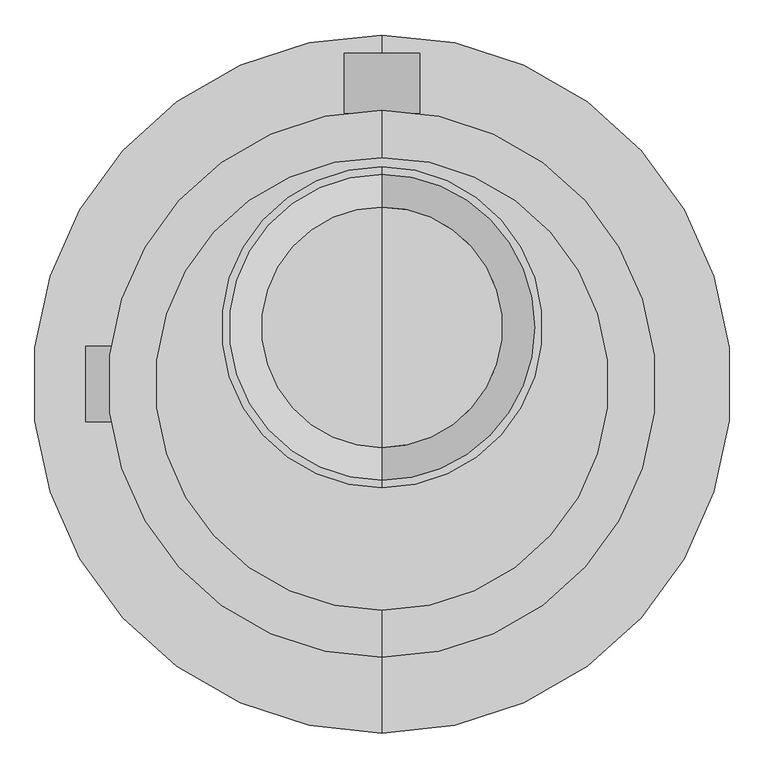
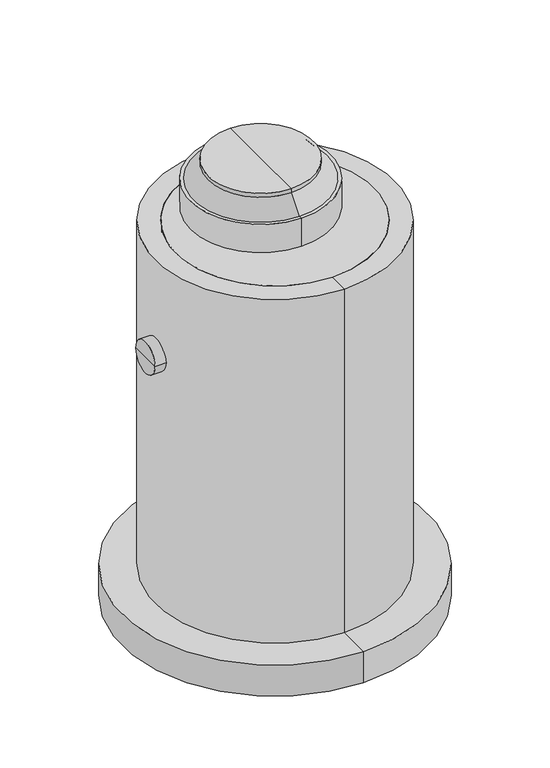
"""IFC4 building model written with IfcOpenShell, lengths in millimetres: proxy geometry, Stormceptor STC - 450 : Stormceptor STC - 450."""

from ifc_helpers import new_model, si_unit, point, frame, origin, origin_2d, place, context, project, spatial, polyline, circle_curve, trimmed, segment, composite_curve, outline, extrude, source, transform, mapped, element, save
from ifc_brep_helpers import plane_surface, cylinder_surface, revolved_surface, advanced_brep


def generic_models_1f94928f(model_context):
    return source(origin(), model_context, "Body", "SolidModel", [
        advanced_brep(
        [(-600.2627198, -101.6, 1828.8), (-600.2627198, 101.6, 1828.8), (-600.2627198, 0.0, 1828.8), (-797.6860951, -101.6, 1828.8), (-797.6860951, 101.6, 1828.8), (-797.6860951, 0.0, 1828.8)],
        [
            (0, 1, circle_curve(frame((-600.2627198, 0.0, 1828.8), z_axis=(1.0, 0.0, 0.0), x_axis=(0.0, 1.0, 0.0)), 101.6)),
            (1, 2),
            (2, 0),
            (1, 0, circle_curve(frame((-600.2627198, 0.0, 1828.8), z_axis=(1.0, 0.0, 0.0), x_axis=(0.0, 1.0, 0.0)), 101.6)),
            (3, 4, circle_curve(frame((-797.6860951, 0.0, 1828.8), z_axis=(1.0, 0.0, 0.0), x_axis=(0.0, 1.0, 0.0)), 101.6)),
            (4, 1),
            (0, 3),
            (4, 3, circle_curve(frame((-797.6860951, 0.0, 1828.8), z_axis=(1.0, 0.0, 0.0), x_axis=(0.0, 1.0, 0.0)), 101.6)),
            (5, 4),
            (3, 5),
        ],
        [
            plane_surface(frame((-600.2627198, 0.0, 1828.8), z_axis=(1.0, 0.0, 0.0), x_axis=(0.0, 1.0, 0.0))),
            cylinder_surface(frame((-1135.9594561, 0.0, 1828.8), z_axis=(-1.0, 0.0, 0.0), x_axis=(0.0, 1.0, 0.0)), 101.6),
            plane_surface(frame((-797.6860951, 0.0, 1828.8), z_axis=(-1.0, 0.0, 0.0), x_axis=(0.0, 1.0, 0.0))),
        ],
        [
            (0, [[1, 2, 3]]),
            (0, [[4, -3, -2]]),
            (1, [[5, 6, -1, 7]]),
            (1, [[8, -7, -4, -6]]),
            (2, [[9, -5, 10]]),
            (2, [[-10, -8, -9]]),
        ],
    ),
        advanced_brep(
        [(-101.6, 729.5594561, 1905.0), (101.6, 729.5594561, 1905.0), (0.0, 729.5594561, 1905.0), (-101.6, 890.1336251, 1905.0), (101.6, 890.1336251, 1905.0), (0.0, 890.1336251, 1905.0)],
        [
            (0, 1, circle_curve(frame((0.0, 729.5594561, 1905.0), z_axis=(0.0, -1.0, 0.0), x_axis=(1.0, 0.0, 0.0)), 101.6)),
            (1, 2),
            (2, 0),
            (1, 0, circle_curve(frame((0.0, 729.5594561, 1905.0), z_axis=(0.0, -1.0, 0.0), x_axis=(1.0, 0.0, 0.0)), 101.6)),
            (3, 4, circle_curve(frame((0.0, 890.1336251, 1905.0), z_axis=(0.0, -1.0, 0.0), x_axis=(1.0, 0.0, 0.0)), 101.6)),
            (4, 1),
            (0, 3),
            (4, 3, circle_curve(frame((0.0, 890.1336251, 1905.0), z_axis=(0.0, -1.0, 0.0), x_axis=(1.0, 0.0, 0.0)), 101.6)),
            (5, 4),
            (3, 5),
        ],
        [
            plane_surface(frame((0.0, 729.5594561, 1905.0), z_axis=(0.0, -1.0, 0.0), x_axis=(1.0, 0.0, 0.0))),
            cylinder_surface(frame((0.0, 805.7594561, 1905.0), z_axis=(0.0, 1.0, 0.0), x_axis=(1.0, 0.0, 0.0)), 101.6),
            plane_surface(frame((0.0, 890.1336251, 1905.0), z_axis=(0.0, 1.0, 0.0), x_axis=(1.0, 0.0, 0.0))),
        ],
        [
            (0, [[1, 2, 3]]),
            (0, [[4, -3, -2]]),
            (1, [[5, 6, -1, 7]]),
            (1, [[8, -7, -4, -6]]),
            (2, [[9, -5, 10]]),
            (2, [[-10, -8, -9]]),
        ],
    ),
        extrude(outline(composite_curve([segment(trimmed(circle_curve(origin_2d(), 609.6), [point((0.0, -609.6))], [point((0.0, 609.6))], False, "CARTESIAN"), True, "CONTINUOUS"), segment(trimmed(circle_curve(origin_2d(), 609.6), [point((0.0, 609.6))], [point((0.0, -609.6))], False, "CARTESIAN"), True, "CONTINUOUS")], self_intersect=False)), frame((0.0, 0.0, 2235.2), z_axis=(0.0, 0.0, 1.0), x_axis=(1.0, 0.0, 0.0)), (0.0, 0.0, 1.0), 203.2),
        advanced_brep(
        [(0.0, 584.2, 2621.28), (0.0, -279.4, 2621.28), (0.0, 152.4, 2621.28), (0.0, 584.2, 2438.4), (0.0, -279.4, 2438.4), (0.0, 152.4, 2438.4)],
        [
            (0, 1, circle_curve(frame((0.0, 152.4, 2621.28), z_axis=(0.0, 0.0, 1.0), x_axis=(0.0, -1.0, 0.0)), 431.8)),
            (1, 2),
            (2, 0),
            (1, 0, circle_curve(frame((0.0, 152.4, 2621.28), z_axis=(0.0, 0.0, 1.0), x_axis=(0.0, -1.0, 0.0)), 431.8)),
            (3, 4, circle_curve(frame((0.0, 152.4, 2438.4), z_axis=(0.0, 0.0, 1.0), x_axis=(0.0, -1.0, 0.0)), 431.8)),
            (4, 1),
            (0, 3),
            (4, 3, circle_curve(frame((0.0, 152.4, 2438.4), z_axis=(0.0, 0.0, 1.0), x_axis=(0.0, -1.0, 0.0)), 431.8)),
            (5, 4),
            (3, 5),
        ],
        [
            plane_surface(frame((0.0, 152.4, 2621.28), z_axis=(0.0, 0.0, 1.0), x_axis=(0.0, -1.0, 0.0))),
            cylinder_surface(frame((0.0, 152.4, 2529.84), z_axis=(0.0, 0.0, -1.0), x_axis=(0.0, -1.0, 0.0)), 431.8),
            plane_surface(frame((0.0, 152.4, 2438.4), z_axis=(0.0, 0.0, -1.0), x_axis=(0.0, -1.0, 0.0))),
        ],
        [
            (0, [[1, 2, 3]]),
            (0, [[4, -3, -2]]),
            (1, [[5, 6, -1, 7]]),
            (1, [[8, -7, -4, -6]]),
            (2, [[9, -5, 10]]),
            (2, [[-10, -8, -9]]),
        ],
    ),
        advanced_brep(
        [(0.0, 609.6, 203.2), (0.0, -609.6, 203.2), (0.0, -736.6, 203.2), (0.0, 736.6, 203.2), (0.0, 609.6, 2438.4), (0.0, -609.6, 2438.4), (0.0, 736.6, 2438.4), (0.0, -736.6, 2438.4)],
        [
            (0, 1, circle_curve(frame((0.0, 0.0, 203.2), z_axis=(0.0, 0.0, 1.0), x_axis=(0.0, -1.0, 0.0)), 609.6)),
            (1, 2),
            (2, 3, circle_curve(frame((0.0, 0.0, 203.2), z_axis=(0.0, 0.0, -1.0), x_axis=(0.0, -1.0, 0.0)), 736.6)),
            (3, 0),
            (1, 0, circle_curve(frame((0.0, 0.0, 203.2), z_axis=(0.0, 0.0, 1.0), x_axis=(0.0, -1.0, 0.0)), 609.6)),
            (3, 2, circle_curve(frame((0.0, 0.0, 203.2), z_axis=(0.0, 0.0, -1.0), x_axis=(0.0, -1.0, 0.0)), 736.6)),
            (4, 5, circle_curve(frame((0.0, 0.0, 2438.4), z_axis=(0.0, 0.0, 1.0), x_axis=(0.0, -1.0, 0.0)), 609.6)),
            (5, 1),
            (0, 4),
            (5, 4, circle_curve(frame((0.0, 0.0, 2438.4), z_axis=(0.0, 0.0, 1.0), x_axis=(0.0, -1.0, 0.0)), 609.6)),
            (6, 7, circle_curve(frame((0.0, 0.0, 2438.4), z_axis=(0.0, 0.0, 1.0), x_axis=(0.0, -1.0, 0.0)), 736.6)),
            (7, 5),
            (4, 6),
            (7, 6, circle_curve(frame((0.0, 0.0, 2438.4), z_axis=(0.0, 0.0, 1.0), x_axis=(0.0, -1.0, 0.0)), 736.6)),
            (2, 7),
            (6, 3),
        ],
        [
            plane_surface(frame((0.0, 0.0, 203.2), z_axis=(0.0, 0.0, -1.0), x_axis=(0.0, -1.0, 0.0))),
            revolved_surface(polyline([(0.0, -609.6, 203.2), (0.0, -609.6, 2438.4)]), (0.0, 0.0, 431.8), (0.0, 0.0, -1.0)),
            plane_surface(frame((0.0, 0.0, 2438.4), z_axis=(0.0, 0.0, 1.0), x_axis=(0.0, -1.0, 0.0))),
            cylinder_surface(frame((0.0, 0.0, 431.8), z_axis=(0.0, 0.0, -1.0), x_axis=(0.0, -1.0, 0.0)), 736.6),
        ],
        [
            (0, [[1, 2, 3, 4]]),
            (0, [[5, -4, 6, -2]]),
            (1, [[7, 8, -1, 9]]),
            (1, [[10, -9, -5, -8]]),
            (2, [[11, 12, -7, 13]]),
            (2, [[14, -13, -10, -12]]),
            (3, [[-3, 15, -11, 16]]),
            (3, [[-6, -16, -14, -15]]),
        ],
    ),
        advanced_brep(
        [(0.0, -171.45, 2722.88), (0.0, 476.25, 2722.88), (0.0, 564.5695326, 2621.28), (0.0, -259.7695326, 2621.28), (0.0, -171.45, 2748.28), (0.0, 476.25, 2748.28), (0.0, 152.4, 2748.28), (0.0, 152.4, 2621.28)],
        [
            (0, 1, circle_curve(frame((0.0, 152.4, 2722.88), z_axis=(0.0, 0.0, -1.0), x_axis=(0.0, 1.0, 0.0)), 323.85)),
            (1, 2),
            (2, 3, circle_curve(frame((0.0, 152.4, 2621.28), z_axis=(0.0, 0.0, 1.0), x_axis=(0.0, 1.0, 0.0)), 412.1695326)),
            (3, 0),
            (1, 0, circle_curve(frame((0.0, 152.4, 2722.88), z_axis=(0.0, 0.0, -1.0), x_axis=(0.0, 1.0, 0.0)), 323.85)),
            (3, 2, circle_curve(frame((0.0, 152.4, 2621.28), z_axis=(0.0, 0.0, 1.0), x_axis=(0.0, 1.0, 0.0)), 412.1695326)),
            (4, 5, circle_curve(frame((0.0, 152.4, 2748.28), z_axis=(0.0, 0.0, -1.0), x_axis=(0.0, 1.0, 0.0)), 323.85)),
            (5, 1),
            (0, 4),
            (5, 4, circle_curve(frame((0.0, 152.4, 2748.28), z_axis=(0.0, 0.0, -1.0), x_axis=(0.0, 1.0, 0.0)), 323.85)),
            (6, 5),
            (4, 6),
            (2, 7),
            (7, 3),
        ],
        [
            revolved_surface(polyline([(0.0, 564.5695326, 2621.28), (0.0, 476.25, 2722.88)]), (0.0, 152.4, 2621.28), (0.0, 0.0, 1.0)),
            cylinder_surface(frame((0.0, 152.4, 2621.28), z_axis=(0.0, 0.0, 1.0), x_axis=(0.0, 1.0, 0.0)), 323.85),
            plane_surface(frame((0.0, 152.4, 2748.28), z_axis=(0.0, 0.0, 1.0), x_axis=(0.0, 1.0, 0.0))),
            plane_surface(frame((0.0, 152.4, 2621.28), z_axis=(0.0, 0.0, -1.0), x_axis=(0.0, 1.0, 0.0))),
        ],
        [
            (0, [[1, 2, 3, 4]]),
            (0, [[5, -4, 6, -2]]),
            (1, [[7, 8, -1, 9]]),
            (1, [[10, -9, -5, -8]]),
            (2, [[11, -7, 12]]),
            (2, [[-12, -10, -11]]),
            (3, [[-3, 13, 14]]),
            (3, [[-6, -14, -13]]),
        ],
    ),
        advanced_brep(
        [(0.0, -939.8, 0.0), (0.0, 939.8, 0.0), (0.0, 0.0, 0.0), (0.0, -939.8, 203.2), (0.0, 939.8, 203.2), (0.0, 0.0, 203.2)],
        [
            (0, 1, circle_curve(frame((0.0, 0.0, 0.0), z_axis=(0.0, 0.0, -1.0), x_axis=(0.0, 1.0, 0.0)), 939.8)),
            (1, 2),
            (2, 0),
            (1, 0, circle_curve(frame((0.0, 0.0, 0.0), z_axis=(0.0, 0.0, -1.0), x_axis=(0.0, 1.0, 0.0)), 939.8)),
            (3, 4, circle_curve(frame((0.0, 0.0, 203.2), z_axis=(0.0, 0.0, -1.0), x_axis=(0.0, 1.0, 0.0)), 939.8)),
            (4, 1),
            (0, 3),
            (4, 3, circle_curve(frame((0.0, 0.0, 203.2), z_axis=(0.0, 0.0, -1.0), x_axis=(0.0, 1.0, 0.0)), 939.8)),
            (5, 4),
            (3, 5),
        ],
        [
            plane_surface(frame((0.0, 0.0, 0.0), z_axis=(0.0, 0.0, -1.0), x_axis=(0.0, 1.0, 0.0))),
            cylinder_surface(frame((0.0, 0.0, 0.0), z_axis=(0.0, 0.0, 1.0), x_axis=(0.0, 1.0, 0.0)), 939.8),
            plane_surface(frame((0.0, 0.0, 203.2), z_axis=(0.0, 0.0, 1.0), x_axis=(0.0, 1.0, 0.0))),
        ],
        [
            (0, [[1, 2, 3]]),
            (0, [[4, -3, -2]]),
            (1, [[5, 6, -1, 7]]),
            (1, [[8, -7, -4, -6]]),
            (2, [[9, -5, 10]]),
            (2, [[-10, -8, -9]]),
        ],
    ),
    ])


if __name__ == "__main__":
    model = new_model("IFC4")
    model_context = context("Model", 3, world=origin())
    ifc_project = project(units=[si_unit("LENGTHUNIT", "METRE", prefix="MILLI")], contexts=[model_context])
    site = spatial("IfcSite", under=ifc_project)
    building = spatial("IfcBuilding", under=site)
    placement = place(None, origin())
    generic_models_shape = generic_models_1f94928f(model_context)
    element("IfcBuildingElementProxy", 1, Name="Stormceptor STC - 450 : Stormceptor STC - 450", ObjectType="Stormceptor STC - 450 : Stormceptor STC - 450", at=placement, inside=building, context=model_context, shape_type="MappedRepresentation", body=[
        mapped(generic_models_shape, transform((0.0, 0.0, 0.0), x_axis=(1.0, 0.0, 0.0), y_axis=(0.0, 1.0, 0.0), z_axis=(0.0, 0.0, 1.0))),
    ])
    save(model, "model.ifc")
